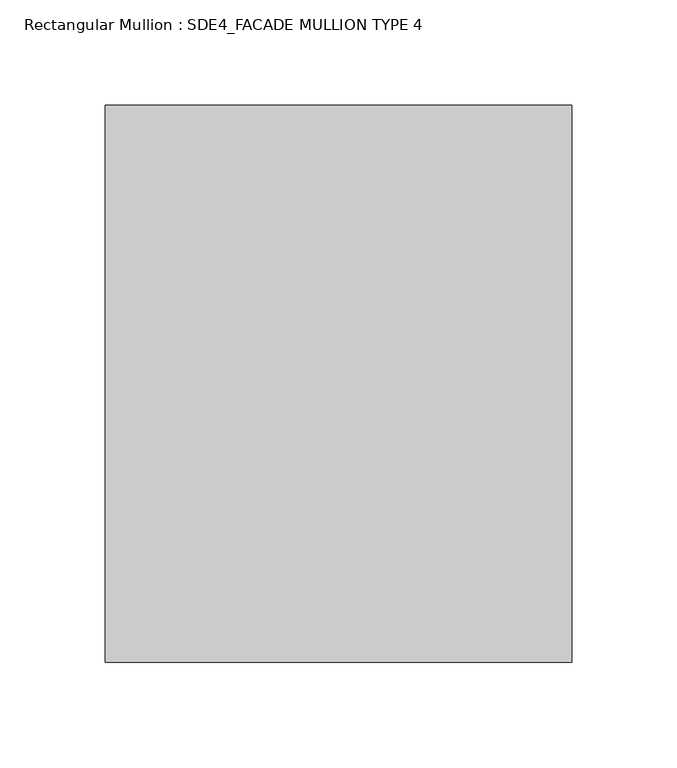
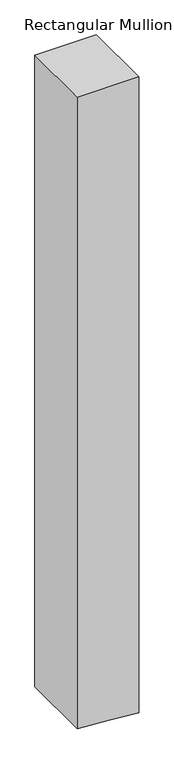
"""IFC4 building model written with IfcOpenShell, lengths in millimetres: member geometry, Rectangular Mullion : SDE4_FACADE MULLION TYPE 4."""

from ifc_helpers import new_model, si_unit, frame, origin, place, context, project, spatial, polyline, outline, extrude, source, transform, mapped, element, save


def rectangular_mullion_sde4_facade_mullion_type_4_9ec5ec8a(model_context):
    return source(origin(), model_context, "Body", "SweptSolid", [
        extrude(outline(polyline([(0.0, 111.0), (0.0, -111.0), (-2413.6224732, -111.0), (-2422.3633948, 3.056508), (-2430.6358347, 111.0), (0.0, 111.0)])), frame((0.0, -132.5, 0.0), z_axis=(0.0, 1.0, 0.0), x_axis=(0.0, 0.0, 1.0)), (0.0, 0.0, 1.0), 265.0),
    ])


if __name__ == "__main__":
    model = new_model("IFC4")
    model_context = context("Model", 3, world=origin())
    ifc_project = project(units=[si_unit("LENGTHUNIT", "METRE", prefix="MILLI")], contexts=[model_context])
    site = spatial("IfcSite", under=ifc_project)
    building = spatial("IfcBuilding", under=site)
    placement = place(None, origin())
    rectangular_mullion_sde4_facade_mullion_type_4_shape = rectangular_mullion_sde4_facade_mullion_type_4_9ec5ec8a(model_context)
    element("IfcMember", 1, ObjectType="Rectangular Mullion : SDE4_FACADE MULLION TYPE 4", at=placement, inside=building, context=model_context, shape_type="MappedRepresentation", body=[
        mapped(rectangular_mullion_sde4_facade_mullion_type_4_shape, transform((0.0, 0.0, 0.0), x_axis=(1.0, 0.0, 0.0), y_axis=(0.0, 1.0, 0.0), z_axis=(0.0, 0.0, 1.0))),
    ])
    save(model, "model.ifc")

# Revit data of these elements
# Type "Rectangular Mullion : SDE4_FACADE MULLION TYPE 4"
#   built-in parameter 1007322 = 0.869423 (stored number, unit not read)
#   built-in parameter 1007321 = 0.364173 (stored number, unit not read)
#   built-in parameter 1007320 = 0.364173 (stored number, unit not read)
